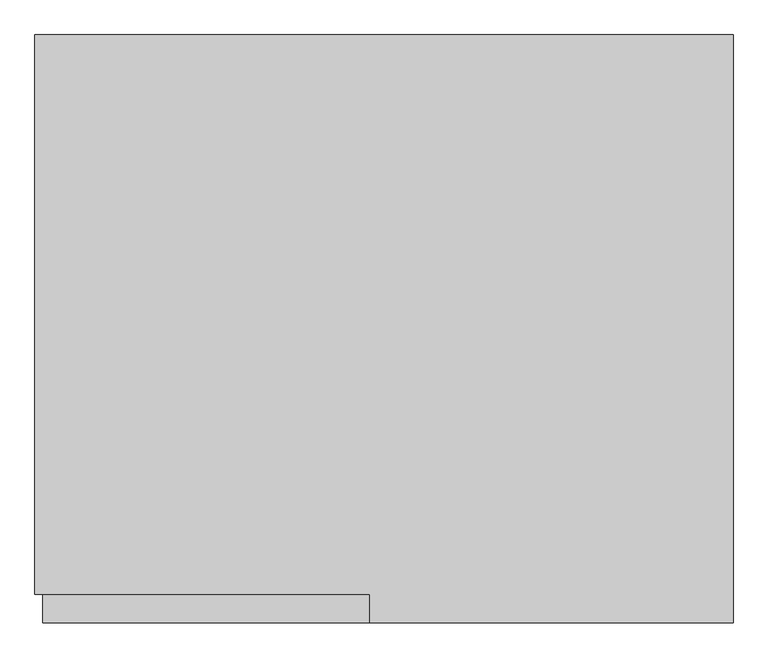
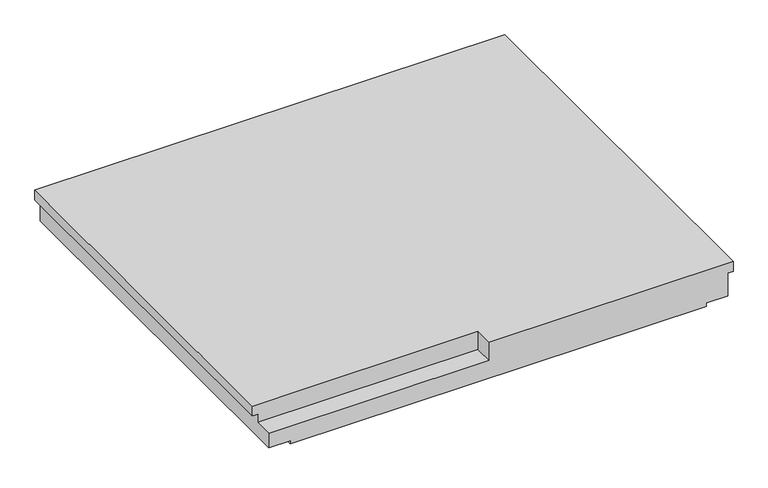
"""IFC4 building model written with IfcOpenShell, lengths in millimetres: proxy geometry, NLRS_24_GM_UN_rechthoekig bordes prefab zonder oplegnok-AV_gen_rsf : prefab bordes_gen__2300x2730."""

from ifc_helpers import new_model, si_unit, origin, place, context, project, spatial, faceted_brep, source, transform, mapped, element, save


def generic_models_f79be4d1(model_context):
    return source(origin(), model_context, "Body", "Brep", [
        faceted_brep([(1365.0, -2300.0, 0.0), (1365.0, -2300.0, -60.0), (1365.0, 0.0, -60.0), (1365.0, 0.0, 0.0), (-55.0, -2300.0, 0.0), (-55.0, -2190.0, 0.0), (-55.0, -2190.0, -110.0), (-55.0, -2300.0, -110.0), (-1365.0, 0.0, 0.0), (-1365.0, 0.0, -60.0), (-1365.0, -2190.0, -60.0), (-1365.0, -2190.0, 0.0), (-1335.0, -2300.0, -110.0), (-1335.0, -2300.0, -200.0), (-1210.0, -2300.0, -200.0), (-1210.0, -2300.0, -220.0), (1210.0, -2300.0, -220.0), (1210.0, -2300.0, -200.0), (1335.0, -2300.0, -200.0), (1335.0, -2300.0, -60.0), (-1335.0, -2190.0, -110.0), (-1335.0, -2190.0, -60.0), (1335.0, 0.0, -60.0), (1335.0, 0.0, -200.0), (1210.0, 0.0, -200.0), (1210.0, 0.0, -220.0), (-1210.0, 0.0, -220.0), (-1210.0, 0.0, -200.0), (-1335.0, 0.0, -200.0), (-1335.0, 0.0, -60.0)], [[[0, 1, 2, 3]], [[4, 5, 6, 7]], [[8, 9, 10, 11]], [[12, 13, 14, 15, 16, 17, 18, 19, 1, 0, 4, 7]], [[7, 6, 20, 12]], [[11, 10, 21, 20, 6, 5]], [[11, 5, 4, 0, 3, 8]], [[8, 3, 2, 22, 23, 24, 25, 26, 27, 28, 29, 9]], [[26, 25, 16, 15]], [[21, 10, 9, 29]], [[13, 12, 20, 21, 29, 28]], [[28, 27, 14, 13]], [[27, 26, 15, 14]], [[22, 2, 1, 19]], [[19, 18, 23, 22]], [[18, 17, 24, 23]], [[17, 16, 25, 24]]]),
    ])


if __name__ == "__main__":
    model = new_model("IFC4")
    model_context = context("Model", 3, world=origin())
    ifc_project = project(units=[si_unit("LENGTHUNIT", "METRE", prefix="MILLI")], contexts=[model_context])
    site = spatial("IfcSite", under=ifc_project)
    building = spatial("IfcBuilding", under=site)
    placement = place(None, origin())
    generic_models_shape = generic_models_f79be4d1(model_context)
    element("IfcBuildingElementProxy", 1, Name="NLRS_24_GM_UN_rechthoekig bordes prefab zonder oplegnok-AV_gen_rsf : prefab bordes_gen__2300x2730", ObjectType="NLRS_24_GM_UN_rechthoekig bordes prefab zonder oplegnok-AV_gen_rsf : prefab bordes_gen__2300x2730", at=placement, inside=building, context=model_context, shape_type="MappedRepresentation", body=[
        mapped(generic_models_shape, transform((0.0, 0.0, 0.0), x_axis=(1.0, 0.0, 0.0), y_axis=(0.0, 1.0, 0.0), z_axis=(0.0, 0.0, 1.0))),
    ])
    save(model, "model.ifc")

# Revit data of these elements
# Type "NLRS_24_GM_UN_rechthoekig bordes prefab zonder oplegnok-AV_gen_rsf : prefab bordes_gen__2300x2730"
#   Export Type to IFC As = "IfcStair"
#   Type IfcGUID = "2CEqVLPNH8KRN7ghwV3a_c"
#   Type Comments = " "
#   Model = " "
#   Manufacturer = " "
#   Description = "rechthoekig bordes prefab\r\n1930x4395"
#   Assembly Code = "24.15"
#   Width = 2730 mm
#   Thickness = 220 mm
#   Perimeter = 10060 mm
#   NLRS_C_lengte_02 = 1310 mm
#   NLRS_C_lengte_01 = 1310 mm
#   NLRS_C_hoogte_02 = 110 mm
#   NLRS_C_hoogte_01 = 110 mm
#   NLRS_C_diepte_04 = 2300 mm
#   NLRS_C_diepte_03 = 2300 mm
#   NLRS_C_diepte_02 = 110 mm
#   NLRS_C_diepte_01 = 110 mm
#   Length = 2300 mm
#   Default Elevation = 1219.2 mm
#   Area = 6.279 m²
#   NLRS_C_materiaal = NLRS_f2_beton prefab_gen_rsf
#   Keynote = ""
# Element 1 (IfcBuildingElementProxy, "NLRS_24_GM_UN_rechthoekig bordes prefab zonder oplegnok-AV_gen_rsf : prefab bordes_gen__2300x2730")
#   Materials on its faces: "NLRS_f2_beton prefab_gen_rsf"
# Materials
#   "NLRS_f2_beton prefab_gen_rsf": class "F - Niet gebakken kunststeen", colour RGB 129 133 118, transparency 0, Keynote = "f2", Manufacturer = "Revit Standards Foundation", URL = "www.revitstandards.org", Description = "beton prefab", Cost = 0
